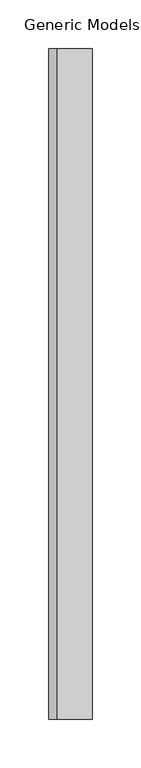
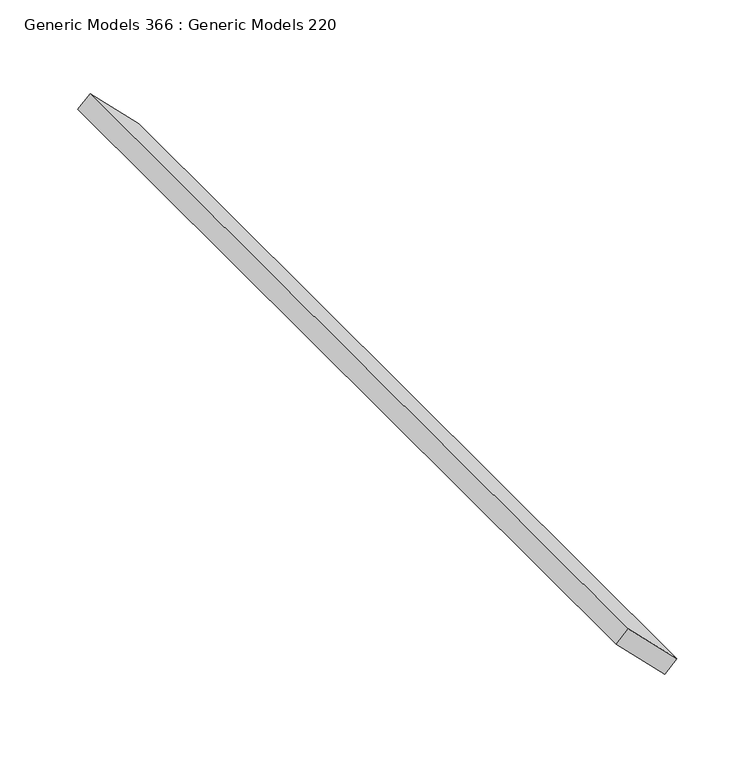
"""IFC4 building model written with IfcOpenShell, lengths in millimetres: proxy geometry, Generic Models 366 : Generic Models 220."""

from ifc_helpers import new_model, si_unit, frame, origin, place, context, project, spatial, polyline, outline, extrude, source, transform, mapped, element, save


def generic_models_366_generic_models_220_cf5c48b1(model_context):
    return source(origin(), model_context, "Body", "SweptSolid", [
        extrude(outline(polyline([(0.0, -50.8), (0.0, 0.0), (690.8142348, 0.0), (690.8142348, -50.8), (0.0, -50.8)])), frame((-6899.085451, -4564.8872686, 128323.1762561), z_axis=(0.7071067811865582, 0.0, 0.7071067811865369), x_axis=(0.0, 1.0, 0.0)), (0.0, 0.0, 1.0), 12.7),
    ])


if __name__ == "__main__":
    model = new_model("IFC4")
    model_context = context("Model", 3, world=origin())
    ifc_project = project(units=[si_unit("LENGTHUNIT", "METRE", prefix="MILLI")], contexts=[model_context])
    site = spatial("IfcSite", under=ifc_project)
    building = spatial("IfcBuilding", under=site)
    placement = place(None, origin())
    generic_models_366_generic_models_220_shape = generic_models_366_generic_models_220_cf5c48b1(model_context)
    element("IfcBuildingElementProxy", 1, Name="Generic Models 366 : Generic Models 220", ObjectType="Generic Models 366 : Generic Models 220", at=placement, inside=building, context=model_context, shape_type="MappedRepresentation", body=[
        mapped(generic_models_366_generic_models_220_shape, transform((0.0, 0.0, 0.0), x_axis=(1.0, 0.0, 0.0), y_axis=(0.0, 1.0, 0.0), z_axis=(0.0, 0.0, 1.0))),
    ])
    save(model, "model.ifc")

# Revit data of these elements
# Element 1 (IfcBuildingElementProxy, "Generic Models 366 : Generic Models 220")
#   Materials on its faces: "_WOOD TONE ALUMINUM EXTRUSION SLAT BY KNOTWOOD"
# Materials
#   "_WOOD TONE ALUMINUM EXTRUSION SLAT BY KNOTWOOD": class "Generic", colour RGB 177 130 114, transparency 0, Cost = 0
